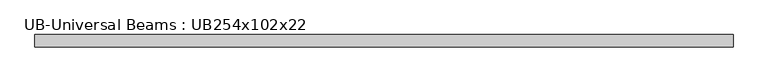
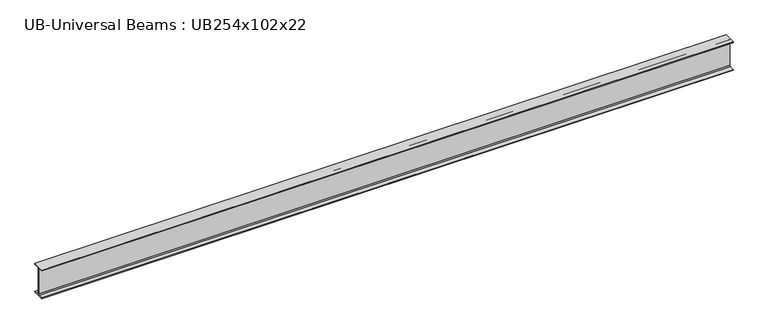
"""IFC4 building model written with IfcOpenShell, lengths in millimetres: beam geometry, UB-Universal Beams : UB254x102x22."""

from ifc_helpers import new_model, si_unit, point, frame, frame_2d, origin, place, context, project, spatial, polyline, circle_curve, trimmed, segment, composite_curve, outline, extrude, source, transform, mapped, element, save


def ub_universal_beams_ub254x102x22_ea344768(model_context):
    return source(origin(), model_context, "Body", "SweptSolid", [
        extrude(outline(composite_curve([segment(polyline([(50.8, -120.2), (50.8, -127.0), (-50.8, -127.0), (-50.8, -120.2), (-10.45, -120.2)]), True, "CONTINUOUS"), segment(trimmed(circle_curve(frame_2d((-10.45, -112.6)), 7.6), [point((-10.45, -120.2))], [point((-2.85, -112.6))], True, "CARTESIAN"), True, "CONTINUOUS"), segment(polyline([(-2.85, -112.6), (-2.85, 112.6)]), True, "CONTINUOUS"), segment(trimmed(circle_curve(frame_2d((-10.45, 112.6)), 7.6), [point((-2.85, 112.6))], [point((-10.45, 120.2))], True, "CARTESIAN"), True, "CONTINUOUS"), segment(polyline([(-10.45, 120.2), (-50.8, 120.2), (-50.8, 127.0), (50.8, 127.0), (50.8, 120.2), (10.45, 120.2)]), True, "CONTINUOUS"), segment(trimmed(circle_curve(frame_2d((10.45, 112.6)), 7.6), [point((10.45, 120.2))], [point((2.85, 112.6))], True, "CARTESIAN"), True, "CONTINUOUS"), segment(polyline([(2.85, 112.6), (2.85, -112.6)]), True, "CONTINUOUS"), segment(trimmed(circle_curve(frame_2d((10.45, -112.6)), 7.6), [point((2.85, -112.6))], [point((10.45, -120.2))], True, "CARTESIAN"), True, "CONTINUOUS"), segment(polyline([(10.45, -120.2), (50.8, -120.2)]), True, "CONTINUOUS")], self_intersect=False)), frame((-2911.1, 0.0, 0.0), z_axis=(1.0, 0.0, 0.0), x_axis=(0.0, 1.0, 0.0)), (0.0, 0.0, 1.0), 5822.2),
    ])


if __name__ == "__main__":
    model = new_model("IFC4")
    model_context = context("Model", 3, world=origin())
    ifc_project = project(units=[si_unit("LENGTHUNIT", "METRE", prefix="MILLI")], contexts=[model_context])
    site = spatial("IfcSite", under=ifc_project)
    building = spatial("IfcBuilding", under=site)
    placement = place(None, origin())
    ub_universal_beams_ub254x102x22_shape = ub_universal_beams_ub254x102x22_ea344768(model_context)
    element("IfcBeam", 1, ObjectType="UB-Universal Beams : UB254x102x22", at=placement, inside=building, context=model_context, shape_type="MappedRepresentation", body=[
        mapped(ub_universal_beams_ub254x102x22_shape, transform((0.0, 0.0, 0.0), x_axis=(1.0, 0.0, 0.0), y_axis=(0.0, 1.0, 0.0), z_axis=(0.0, 0.0, 1.0))),
    ])
    save(model, "model.ifc")

# Revit data of these elements
# Type "UB-Universal Beams : UB254x102x22"
#   Section Name Key = "UB254X102X22"
#   Width = 10.16 cm
#   Web Thickness = 0.57 cm
#   Web Fillet = 0.76 cm
#   Warping Constant = 18200.0 cm⁶
#   Torsional Moment of Inertia = 4.15 cm⁴
#   Section Area = 28.0 cm²
#   Plastic Modulus weak axis = 37.3 cm³
#   Plastic Modulus strong axis = 259.0 cm³
#   Nominal Weight = 22.00 kgf/m
#   Moment of Inertia weak axis = 119.00 cm⁴
#   Moment of Inertia strong axis = 2841.00 cm⁴
#   Height = 25.4 cm
#   Flange Thickness = 0.68 cm
#   Elastic Modulus weak axis = 23.5 cm³
#   Elastic Modulus strong axis = 224.0 cm³
#   Centroid Vertical = 12.7 cm
#   Centroid Horizontal = 5.08 cm
#   Bolt Spacing = 5.4 cm
#   Length [instance default] = 1500 mm
#   Structural Material [instance default] = Metal - Steel 43-275
#   Type Comments = ""
#   Assembly Code = ""
# Element 1 (IfcBeam, "UB-Universal Beams : UB254x102x22")
#   Materials on its faces: "Metal - Steel 43-275"
# Materials
#   "Metal - Steel 43-275": class "Metal", colour RGB 247 247 247, transparency 0, Cost = 0
